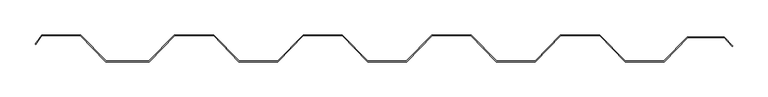
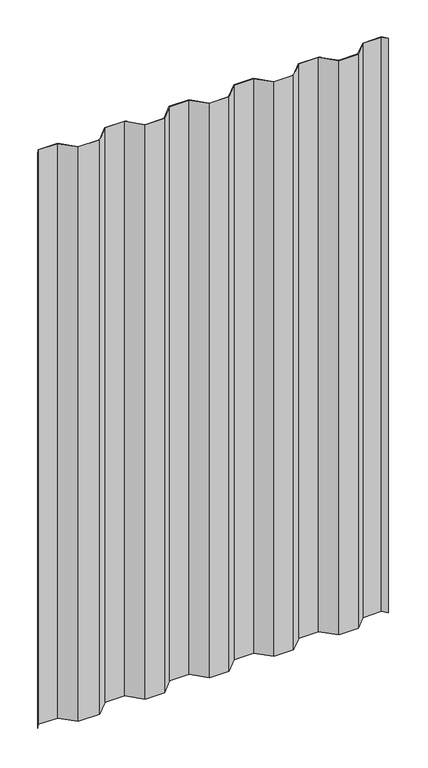
"""IFC4 building model written with IfcOpenShell, lengths in millimetres: proxy geometry, Generic Models 2:Generic Models 2:310765:Generic Models 2:310765 : Generic Models 2:Generic Models 2:310765:19 : Generic Models 2:Generic Models 2:310765:Generic Models 2:310765 : Generic Models 2:Generic Models 2:310765:300385."""

from ifc_helpers import new_model, si_unit, frame, origin, place, context, project, spatial, polyline, outline, extrude, source, transform, mapped, element, save


def generic_models_502fc135(model_context):
    return source(origin(), model_context, "Body", "SweptSolid", [
        extrude(outline(polyline([(570516.8090826, -578743.0895469), (570528.6648289, -578756.1976179), (570528.1028571, -578756.7595897), (570516.4567453, -578743.8832969), (570464.5503913, -578743.8832969), (570430.9184065, -578778.4413841), (570375.7388466, -578778.4413841), (570339.5766549, -578741.1351341), (570284.2015293, -578741.1351341), (570248.0393377, -578778.4413841), (570192.8588466, -578778.4413841), (570156.6966549, -578741.1351341), (570101.3215293, -578741.1351341), (570065.1593377, -578778.4413841), (570009.9788466, -578778.4413841), (569973.8166549, -578741.1351341), (569918.4415293, -578741.1351341), (569882.2793377, -578778.4413841), (569827.0988466, -578778.4413841), (569790.9366549, -578741.1351341), (569735.5615293, -578741.1351341), (569699.3993377, -578778.4413841), (569637.8688466, -578778.4413841), (569601.7066549, -578741.1351341), (569547.1780922, -578741.1351341), (569538.2367239, -578753.9047314), (569537.586522, -578753.4494551), (569546.7648921, -578740.3413841), (569602.0427005, -578740.3413841), (569638.2048921, -578777.6476341), (569699.0632921, -578777.6476341), (569735.2254838, -578740.3413841), (569791.2727005, -578740.3413841), (569827.4348921, -578777.6476341), (569881.9432921, -578777.6476341), (569918.1054838, -578740.3413841), (569974.1527005, -578740.3413841), (570010.3148921, -578777.6476341), (570064.8232921, -578777.6476341), (570100.9854838, -578740.3413841), (570157.0327005, -578740.3413841), (570193.1948921, -578777.6476341), (570247.7032921, -578777.6476341), (570283.8654838, -578740.3413841), (570339.9127005, -578740.3413841), (570376.0748921, -578777.6476341), (570430.5832921, -578777.6476341), (570464.2152769, -578743.0895469), (570516.8090826, -578743.0895469)])), frame((0.0, 0.0, 4438.4276051), z_axis=(0.0, 0.0, 1.0), x_axis=(1.0, 0.0, 0.0)), (0.0, 0.0, 1.0), 1717.3793287),
    ])


if __name__ == "__main__":
    model = new_model("IFC4")
    model_context = context("Model", 3, world=origin())
    ifc_project = project(units=[si_unit("LENGTHUNIT", "METRE", prefix="MILLI")], contexts=[model_context])
    site = spatial("IfcSite", under=ifc_project)
    building = spatial("IfcBuilding", under=site)
    placement = place(None, origin())
    generic_models_shape = generic_models_502fc135(model_context)
    element("IfcBuildingElementProxy", 1, Name="Generic Models 2:Generic Models 2:310765:Generic Models 2:310765 : Generic Models 2:Generic Models 2:310765:19 : Generic Models 2:Generic Models 2:310765:Generic Models 2:310765 : Generic Models 2:Generic Models 2:310765:300385", ObjectType="Generic Models 2:Generic Models 2:310765:Generic Models 2:310765 : Generic Models 2:Generic Models 2:310765:19 : Generic Models 2:Generic Models 2:310765:Generic Models 2:310765 : Generic Models 2:Generic Models 2:310765:300385", at=placement, inside=building, context=model_context, shape_type="MappedRepresentation", body=[
        mapped(generic_models_shape, transform((0.0, 0.0, 0.0), x_axis=(1.0, 0.0, 0.0), y_axis=(0.0, 1.0, 0.0), z_axis=(0.0, 0.0, 1.0))),
    ])
    save(model, "model.ifc")

# Revit data of these elements
# Type "Generic Models 2:Generic Models 2:310765:Generic Models 2:310765 : Generic Models 2:Generic Models 2:310765:19 : Generic Models 2:Generic Models 2:310765:Generic Models 2:310765 : Generic Models 2:Generic Models 2:310765:300385"
#   NameOverride = "Generic Models 2:Generic Models 2:310765:Generic Models 2:310765 : Generic Models 2:Generic Models 2:310765:300385"
#   ObjectTypeOverride = "Generic Models 2:310765 : Generic Models 2:Generic Models 2:310765"
#   Reference = "Generic Models 2"
#   Tag = "300385"
# Element 1 (IfcBuildingElementProxy, "Generic Models 2:Generic Models 2:310765:Generic Models 2:310765 : Generic Models 2:Generic Models 2:310765:19 : Generic Models 2:Generic Models 2:310765:Generic Models 2:310765 : Generic Models 2:Generic Models 2:310765:300385")
#   Materials on its faces: "VERTICAL CORRUGATED METAL PANEL - EXPOSED FASTENERS - (MBCI 7.2 PANEL)"
# Materials
#   "VERTICAL CORRUGATED METAL PANEL - EXPOSED FASTENERS - (MBCI 7.2 PANEL)": class "Generic", colour RGB 120 120 120, transparency 0, Cost = 0
